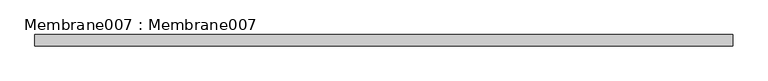
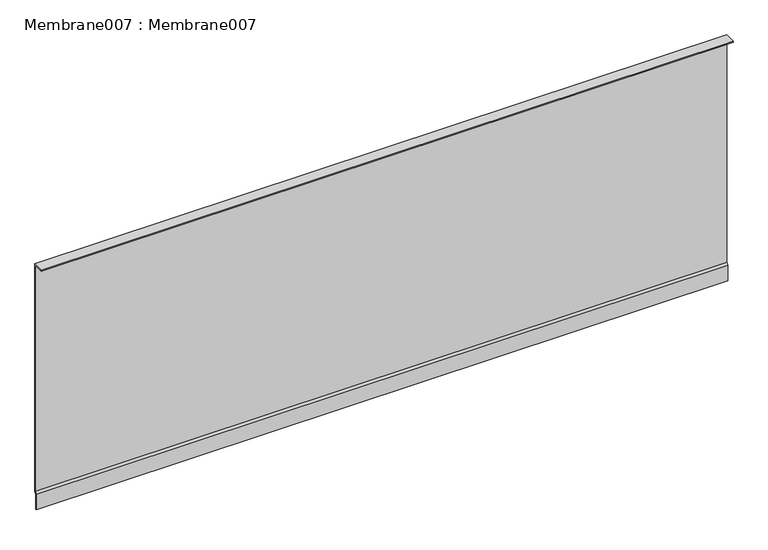
"""IFC4 building model written with IfcOpenShell, lengths in millimetres: proxy geometry, Membrane007 : Membrane007."""

import ifcopenshell
import ifcopenshell.guid

model = None  # the IFC model being written
_history = None  # IfcOwnerHistory: only IFC2X3 demands one
_inside = {}  # id of a spatial element -> (the spatial element, [elements in it])
_under = {}  # id of a project, library or spatial element -> (it, [spatial elements below it])
_declared = {}  # id of a project -> (the project, [libraries it declares])
_typed = {}  # id of a type object -> (the type object, [elements of that type])
_made_of = {}  # id of a material, layer set ... -> (it, [elements and type objects made of it])


def new_model(schema):
    """Start an empty IFC model of exactly this schema.

    Asked for "IFC4X3", IfcOpenShell would pick the latest addendum, in which some entities
    have other attributes; the version numbers below select the first issue.
    IFC2X3 requires an IfcOwnerHistory on every rooted entity: one is made here for all.
    """
    global model, _history
    if schema == "IFC4X3":
        model = ifcopenshell.file(schema_version=(4, 3, 0, 0))
    else:
        model = ifcopenshell.file(schema=schema)
    _inside.clear()
    _under.clear()
    _declared.clear()
    _typed.clear()
    _made_of.clear()
    _history = None
    if model.schema == "IFC2X3":
        org = make("IfcOrganization", Name="unknown")
        user = make(
            "IfcPersonAndOrganization",
            ThePerson=make("IfcPerson", FamilyName="unknown"),
            TheOrganization=org,
        )
        app = make(
            "IfcApplication",
            ApplicationDeveloper=org,
            Version="unknown",
            ApplicationFullName="unknown",
            ApplicationIdentifier="unknown",
        )
        _history = make(
            "IfcOwnerHistory",
            OwningUser=user,
            OwningApplication=app,
            ChangeAction="ADDED",
            CreationDate=0,
        )
    return model


def make(cls, **values):
    """One entity of the class cls with the attributes given. An attribute that is None is left unset."""
    return model.create_entity(
        cls, **{name: value for name, value in values.items() if value is not None}
    )


def rooted(cls, **values):
    """An entity with a GlobalId (a new one), such as an element, a storey or a relation."""
    return make(cls, GlobalId=ifcopenshell.guid.new(), OwnerHistory=_history, **values)


def si_unit(unit_type, name, prefix=None):
    """IfcSIUnit, for example si_unit("LENGTHUNIT", "METRE", prefix="MILLI")."""
    return make("IfcSIUnit", UnitType=unit_type, Prefix=prefix, Name=name)


def assignment(units):
    """IfcUnitAssignment: the units of a project."""
    return None if units is None else make("IfcUnitAssignment", Units=units)


def point(xyz):
    """IfcCartesianPoint."""
    return None if xyz is None else make("IfcCartesianPoint", Coordinates=xyz)


def direction(xyz):
    """IfcDirection."""
    return None if xyz is None else make("IfcDirection", DirectionRatios=xyz)


def frame(location, z_axis=None, x_axis=None):
    """IfcAxis2Placement3D, a coordinate frame: its origin and axes. An axis left out is left unset."""
    return make(
        "IfcAxis2Placement3D",
        Location=point(location),
        Axis=direction(z_axis),
        RefDirection=direction(x_axis),
    )


def origin():
    """The frame at (0, 0, 0) with its axes left unset."""
    return frame((0.0, 0.0, 0.0))


def place(relative_to, where):
    """IfcLocalPlacement: puts the frame where relative to a parent placement (None: the world)."""
    return make(
        "IfcLocalPlacement", PlacementRelTo=relative_to, RelativePlacement=where
    )


def context(
    kind, dimensions, precision=None, world=None, true_north=None, identifier=None
):
    """IfcGeometricRepresentationContext, for example the 3D "Model" context."""
    return make(
        "IfcGeometricRepresentationContext",
        ContextIdentifier=identifier,
        ContextType=kind,
        CoordinateSpaceDimension=dimensions,
        Precision=precision,
        WorldCoordinateSystem=world,
        TrueNorth=true_north,
    )


def project(units=None, contexts=None):
    """IfcProject with its units and contexts."""
    return rooted(
        "IfcProject",
        Name="project",
        RepresentationContexts=contexts,
        UnitsInContext=assignment(units),
    )


def spatial(cls, under=None, at=None, **own):
    """A site, building, storey or space (cls), placed at a placement, below another one or the project."""
    s = rooted(cls, ObjectPlacement=at, **own)
    if under is not None:
        _under.setdefault(under.id(), (under, []))[1].append(s)
    return s


def polyline(points):
    """IfcPolyline through the points."""
    return make("IfcPolyline", Points=[point(p) for p in points])


def outline(outer, holes=None, kind="AREA"):
    """IfcArbitraryClosedProfileDef: a profile drawn as a closed curve; with holes, ...WithVoids."""
    if holes is None:
        return make("IfcArbitraryClosedProfileDef", ProfileType=kind, OuterCurve=outer)
    return make(
        "IfcArbitraryProfileDefWithVoids",
        ProfileType=kind,
        OuterCurve=outer,
        InnerCurves=holes,
    )


def extrude(swept, where, along, depth):
    """IfcExtrudedAreaSolid: the profile swept, set in the frame where, extruded along a direction by depth."""
    return make(
        "IfcExtrudedAreaSolid",
        SweptArea=swept,
        Position=where,
        ExtrudedDirection=direction(along),
        Depth=depth,
    )


def shape(context_of_items, identifier, shape_type, items):
    """IfcShapeRepresentation: the items that make up one representation, for example the "Body"."""
    return make(
        "IfcShapeRepresentation",
        ContextOfItems=context_of_items,
        RepresentationIdentifier=identifier,
        RepresentationType=shape_type,
        Items=items,
    )


def source(mapping_origin, context_of_items, identifier, shape_type, items):
    """IfcRepresentationMap: a shape defined once, which mapped items show again and again."""
    return make(
        "IfcRepresentationMap",
        MappingOrigin=mapping_origin,
        MappedRepresentation=shape(context_of_items, identifier, shape_type, items),
    )


def transform(
    local_origin,
    x_axis=None,
    y_axis=None,
    z_axis=None,
    scale=None,
    scale2=None,
    scale3=None,
    uniform=True,
):
    """IfcCartesianTransformationOperator3D, or its non-uniform kind. x_axis, y_axis, z_axis: its Axis1, 2, 3."""
    if uniform:
        return make(
            "IfcCartesianTransformationOperator3D",
            Axis1=direction(x_axis),
            Axis2=direction(y_axis),
            LocalOrigin=point(local_origin),
            Scale=scale,
            Axis3=direction(z_axis),
        )
    return make(
        "IfcCartesianTransformationOperator3DnonUniform",
        Axis1=direction(x_axis),
        Axis2=direction(y_axis),
        LocalOrigin=point(local_origin),
        Scale=scale,
        Axis3=direction(z_axis),
        Scale2=scale2,
        Scale3=scale3,
    )


def mapped(mapping_source, mapping_target):
    """IfcMappedItem: shows the shape of a source again, moved by a transform."""
    return make(
        "IfcMappedItem", MappingSource=mapping_source, MappingTarget=mapping_target
    )


def made_of(thing, what):
    """Note that an element or type object is made of a material, layer set ...; save() writes the relation."""
    if what is not None:
        _made_of.setdefault(what.id(), (what, []))[1].append(thing)
    return thing


def element(
    cls,
    number,
    at=None,
    inside=None,
    cuts=None,
    type_object=None,
    material=None,
    context=None,
    identifier="Body",
    shape_type=None,
    held_by="IfcProductDefinitionShape",
    body=None,
    shapes=None,
    **own,
):
    """One element of the class cls, such as IfcWall. Its Tag is "e" and its number.

    at: its placement. inside: the storey or other place that contains it. cuts: it is an
    opening in that element (IfcRelVoidsElement). A single representation is given by context,
    identifier, shape_type and body (its items); several are given by shapes. held_by: the class
    of the entity that holds the representations. save() writes the other relations.
    """
    e = rooted(cls, Tag="e%d" % number, ObjectPlacement=at, **own)
    if body is not None:
        shapes = [shape(context, identifier, shape_type, body)]
    if shapes is not None:
        e.Representation = make(held_by, Representations=shapes)
    if inside is not None:
        _inside.setdefault(inside.id(), (inside, []))[1].append(e)
    if cuts is not None:
        rooted(
            "IfcRelVoidsElement", RelatingBuildingElement=cuts, RelatedOpeningElement=e
        )
    if type_object is not None:
        _typed.setdefault(type_object.id(), (type_object, []))[1].append(e)
    return made_of(e, material)


def aggregate(whole, parts):
    """IfcRelAggregates: a whole, such as a stair, and the parts it consists of."""
    return rooted("IfcRelAggregates", RelatingObject=whole, RelatedObjects=parts)


def save(model, path):
    """Write the relations noted so far, then the file.

    IfcRelAggregates (storeys below a building ...), IfcRelContainedInSpatialStructure (elements
    in a storey), IfcRelDefinesByType, IfcRelAssociatesMaterial and IfcRelDeclares: one each for
    every whole, place, type object, material and project.
    """
    for whole, parts in _under.values():
        aggregate(whole, parts)
    for where, things in _inside.values():
        rooted(
            "IfcRelContainedInSpatialStructure",
            RelatedElements=things,
            RelatingStructure=where,
        )
    for kind, things in _typed.values():
        rooted("IfcRelDefinesByType", RelatedObjects=things, RelatingType=kind)
    for what, things in _made_of.values():
        rooted("IfcRelAssociatesMaterial", RelatedObjects=things, RelatingMaterial=what)
    for by, libraries in _declared.values():
        rooted("IfcRelDeclares", RelatingContext=by, RelatedDefinitions=libraries)
    model.write(path)


def membrane007_membrane007_2d422dc0(model_context):
    return source(origin(), model_context, "Body", "SweptSolid", [
        extrude(outline(polyline([(-4691.2641602, 39752.9375), (-4691.2641602, 39754.9375), (-4658.5039063, 39754.9375), (-4658.5039063, 39060.3828125), (-4662.7177734, 39054.1640625), (-4662.7177734, 39007.46875), (-4664.7177734, 39007.46875), (-4664.7177734, 39054.7778498), (-4660.5039062, 39060.9965998), (-4660.5039062, 39752.9375), (-4691.2641602, 39752.9375)])), frame((12383.0178845, 0.0, 0.0), z_axis=(1.0, 0.0, 0.0), x_axis=(0.0, 1.0, 0.0)), (0.0, 0.0, 1.0), 2000.0),
    ])


if __name__ == "__main__":
    model = new_model("IFC4")
    model_context = context("Model", 3, world=origin())
    ifc_project = project(units=[si_unit("LENGTHUNIT", "METRE", prefix="MILLI")], contexts=[model_context])
    site = spatial("IfcSite", under=ifc_project)
    building = spatial("IfcBuilding", under=site)
    placement = place(None, origin())
    membrane007_membrane007_shape = membrane007_membrane007_2d422dc0(model_context)
    element("IfcBuildingElementProxy", 1, Name="Membrane007 : Membrane007", ObjectType="Membrane007 : Membrane007", at=placement, inside=building, context=model_context, shape_type="MappedRepresentation", body=[
        mapped(membrane007_membrane007_shape, transform((0.0, 0.0, 0.0), x_axis=(1.0, 0.0, 0.0), y_axis=(0.0, 1.0, 0.0), z_axis=(0.0, 0.0, 1.0))),
    ])
    save(model, "model.ifc")

# Revit data of these elements
# Type "Membrane007 : Membrane007"
#   NameOverride = "Membrane007"
# Element 1 (IfcBuildingElementProxy, "Membrane007 : Membrane007")
#   Materials on its faces: "2 LAYERS NO. 30 ASTM D226 ASPHALT SATURATED ORGANIC FELT"
# Materials
#   "2 LAYERS NO. 30 ASTM D226 ASPHALT SATURATED ORGANIC FELT": class "Unassigned", colour RGB 46 171 0, transparency 0
